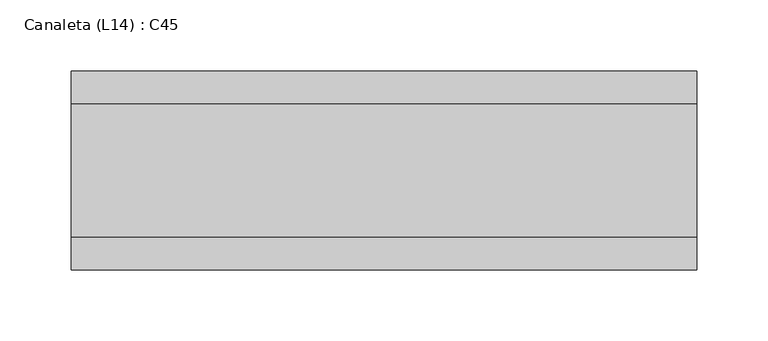
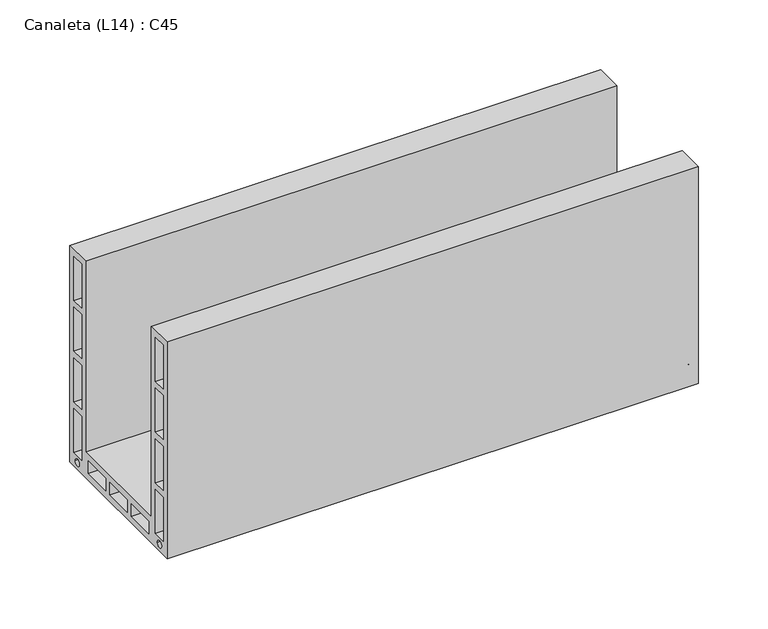
"""IFC4 building model written with IfcOpenShell, lengths in millimetres: proxy geometry, Canaleta (L14) : C45."""

from ifc_helpers import new_model, si_unit, point, frame, frame_2d, origin, place, context, project, spatial, polyline, circle_curve, trimmed, segment, composite_curve, outline, extrude, source, transform, mapped, element, save


def canaleta_l14_c45_c2fd00c5(model_context):
    return source(origin(), model_context, "Body", "SweptSolid", [
        extrude(outline(polyline([(140.0, 0.0), (0.0, 0.0), (0.0, 190.0), (23.0, 190.0), (23.0, 23.0), (117.0, 23.0), (117.0, 190.0), (140.0, 190.0), (140.0, 0.0)]), holes=[polyline([(123.0, 184.0), (123.0, 145.5), (134.0, 145.5), (134.0, 184.0), (123.0, 184.0)]), polyline([(123.0, 139.5), (123.0, 101.0), (134.0, 101.0), (134.0, 139.5), (123.0, 139.5)]), polyline([(123.0, 95.0), (123.0, 56.5), (134.0, 56.5), (134.0, 95.0), (123.0, 95.0)]), polyline([(123.0, 50.5), (123.0, 12.0), (134.0, 12.0), (134.0, 50.5), (123.0, 50.5)]), composite_curve([segment(trimmed(circle_curve(frame_2d((128.9426557, 6.2112346)), 3.0), [point((125.9426557, 6.2112346))], [point((131.9426557, 6.2112346))], True, "CARTESIAN"), True, "CONTINUOUS"), segment(trimmed(circle_curve(frame_2d((128.9426557, 6.2112346)), 3.0), [point((131.9426557, 6.2112346))], [point((125.9426557, 6.2112346))], True, "CARTESIAN"), True, "CONTINUOUS")], self_intersect=False), polyline([(17.0, 184.0), (6.0, 184.0), (6.0, 145.5), (17.0, 145.5), (17.0, 184.0)]), polyline([(17.0, 139.5), (6.0, 139.5), (6.0, 101.0), (17.0, 101.0), (17.0, 139.5)]), polyline([(17.0, 95.0), (6.0, 95.0), (6.0, 56.5), (17.0, 56.5), (17.0, 95.0)]), polyline([(17.0, 50.5), (6.0, 50.5), (6.0, 12.0), (17.0, 12.0), (17.0, 50.5)]), composite_curve([segment(trimmed(circle_curve(frame_2d((11.0573443, 6.2112346)), 3.0), [point((8.0573443, 6.2112346))], [point((14.0573443, 6.2112346))], True, "CARTESIAN"), True, "CONTINUOUS"), segment(trimmed(circle_curve(frame_2d((11.0573443, 6.2112346)), 3.0), [point((14.0573443, 6.2112346))], [point((8.0573443, 6.2112346))], True, "CARTESIAN"), True, "CONTINUOUS")], self_intersect=False), polyline([(88.5, 17.0), (88.5, 6.0), (113.5, 6.0), (113.5, 17.0), (88.5, 17.0)]), polyline([(57.5, 17.0), (57.5, 6.0), (82.5, 6.0), (82.5, 17.0), (57.5, 17.0)]), polyline([(26.5, 17.0), (26.5, 6.0), (51.5, 6.0), (51.5, 17.0), (26.5, 17.0)])]), frame((0.0, 0.0, 0.0), z_axis=(1.0, 0.0, 0.0), x_axis=(0.0, 1.0, 0.0)), (0.0, 0.0, 1.0), 440.0),
    ])


if __name__ == "__main__":
    model = new_model("IFC4")
    model_context = context("Model", 3, world=origin())
    ifc_project = project(units=[si_unit("LENGTHUNIT", "METRE", prefix="MILLI")], contexts=[model_context])
    site = spatial("IfcSite", under=ifc_project)
    building = spatial("IfcBuilding", under=site)
    placement = place(None, origin())
    canaleta_l14_c45_shape = canaleta_l14_c45_c2fd00c5(model_context)
    element("IfcBuildingElementProxy", 1, Name="Canaleta (L14) : C45", ObjectType="Canaleta (L14) : C45", at=placement, inside=building, context=model_context, shape_type="MappedRepresentation", body=[
        mapped(canaleta_l14_c45_shape, transform((0.0, 0.0, 0.0), x_axis=(1.0, 0.0, 0.0), y_axis=(0.0, 1.0, 0.0), z_axis=(0.0, 0.0, 1.0))),
    ])
    save(model, "model.ifc")

# Revit data of these elements
# Type "Canaleta (L14) : C45"
#   Comprimento = 0.440 m
#   Material [instance default] = Blocos Cerâmicos
#   Default Elevation = 0
# Element 1 (IfcBuildingElementProxy, "Canaleta (L14) : C45")
#   Materials on its faces: "Blocos Cerâmicos"
# Materials
#   "Blocos Cerâmicos": class "Genérico", colour RGB 177 84 47, transparency 0, Cost = 0
